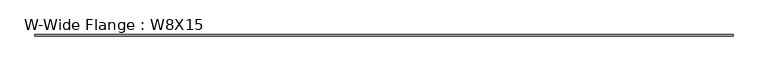
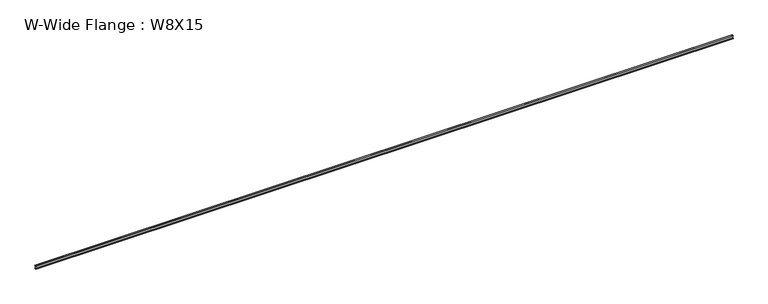
"""IFC4 building model written with IfcOpenShell, lengths in millimetres: beam geometry, W-Wide Flange : W8X15."""

from ifc_helpers import new_model, si_unit, point, frame, frame_2d, origin, place, context, project, spatial, polyline, circle_curve, trimmed, segment, composite_curve, outline, extrude, source, transform, mapped, element, save


def w_wide_flange_w8x15_b0d89ca1(model_context):
    return source(origin(), model_context, "Body", "SweptSolid", [
        extrude(outline(composite_curve([segment(polyline([(50.927, -94.996), (50.927, -102.997), (-50.927, -102.997), (-50.927, -94.996), (-15.748, -94.996)]), True, "CONTINUOUS"), segment(trimmed(circle_curve(frame_2d((-15.748, -82.3595)), 12.6365), [point((-15.748, -94.996))], [point((-3.1115, -82.3595))], True, "CARTESIAN"), True, "CONTINUOUS"), segment(polyline([(-3.1115, -82.3595), (-3.1115, 82.3595)]), True, "CONTINUOUS"), segment(trimmed(circle_curve(frame_2d((-15.748, 82.3595)), 12.6365), [point((-3.1115, 82.3595))], [point((-15.748, 94.996))], True, "CARTESIAN"), True, "CONTINUOUS"), segment(polyline([(-15.748, 94.996), (-50.927, 94.996), (-50.927, 102.997), (50.927, 102.997), (50.927, 94.996), (15.748, 94.996)]), True, "CONTINUOUS"), segment(trimmed(circle_curve(frame_2d((15.748, 82.3595)), 12.6365), [point((15.748, 94.996))], [point((3.1115, 82.3595))], True, "CARTESIAN"), True, "CONTINUOUS"), segment(polyline([(3.1115, 82.3595), (3.1115, -82.3595)]), True, "CONTINUOUS"), segment(trimmed(circle_curve(frame_2d((15.748, -82.3595)), 12.6365), [point((3.1115, -82.3595))], [point((15.748, -94.996))], True, "CARTESIAN"), True, "CONTINUOUS"), segment(polyline([(15.748, -94.996), (50.927, -94.996)]), True, "CONTINUOUS")], self_intersect=False)), frame((-24143.096875, 0.0, 0.0), z_axis=(1.0, 0.0, 0.0), x_axis=(0.0, 1.0, 0.0)), (0.0, 0.0, 1.0), 48120.3),
    ])


if __name__ == "__main__":
    model = new_model("IFC4")
    model_context = context("Model", 3, world=origin())
    ifc_project = project(units=[si_unit("LENGTHUNIT", "METRE", prefix="MILLI")], contexts=[model_context])
    site = spatial("IfcSite", under=ifc_project)
    building = spatial("IfcBuilding", under=site)
    placement = place(None, origin())
    w_wide_flange_w8x15_shape = w_wide_flange_w8x15_b0d89ca1(model_context)
    element("IfcBeam", 1, ObjectType="W-Wide Flange : W8X15", at=placement, inside=building, context=model_context, shape_type="MappedRepresentation", body=[
        mapped(w_wide_flange_w8x15_shape, transform((0.0, 0.0, 0.0), x_axis=(1.0, 0.0, 0.0), y_axis=(0.0, 1.0, 0.0), z_axis=(0.0, 0.0, 1.0))),
    ])
    save(model, "model.ifc")

# Revit data of these elements
# Type "W-Wide Flange : W8X15"
#   Assembly Code = "B10"
#   W = 15
#   Length [instance default] = 5' - 0"
#   bf = 0' - 4.01"
#   d = 0' - 8.11"
#   k = 0' - 0 13/16"
#   k2 = 0' - 0.4975"
#   tf = 0' - 0.315"
#   tw = 0' - 0.245"
#   A = 0.0308333 SF
#   Structural Material [instance default] = Steel ASTM A992
# Element 1 (IfcBeam, "W-Wide Flange : W8X15")
#   Materials on its faces: "Steel ASTM A992"
# Materials
#   "Steel ASTM A992": class "Metal", colour RGB 199 199 199, transparency 0, Description = "Structural steel 50ksi", Cost = 0
